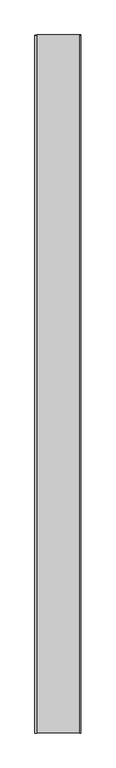
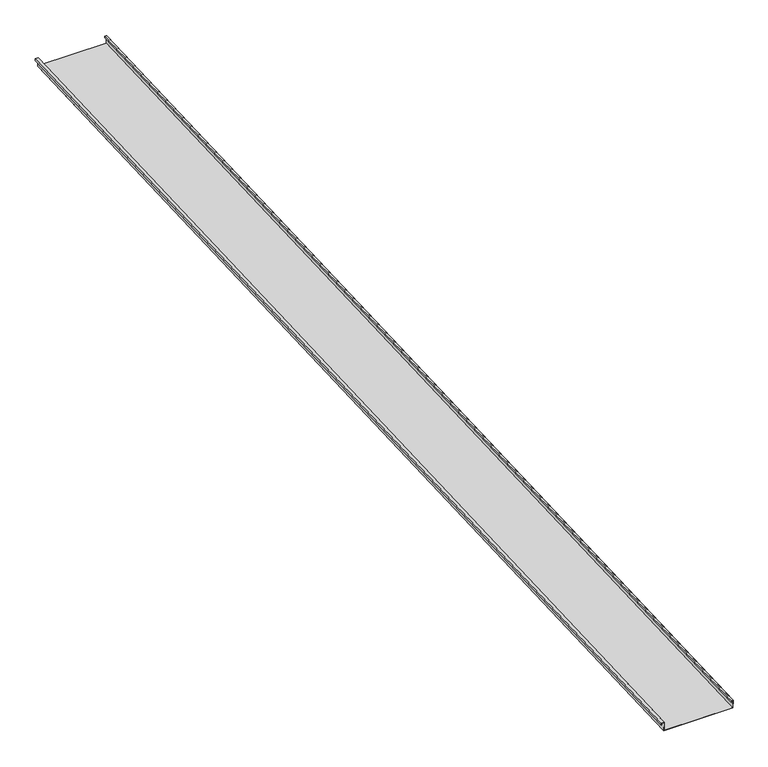
"""IFC4 building model written with IfcOpenShell, lengths in millimetres: proxy geometry, Generic Models 2:Generic Models 2:310765:Generic Models 2:310765 : Generic Models 2:Generic Models 2:310765:98 : Generic Models 2:Generic Models 2:310765:Generic Models 2:310765 : Generic Models 2:Generic Models 2:310765:300385."""

from ifc_helpers import new_model, si_unit, frame, origin, place, context, project, spatial, polyline, outline, extrude, source, transform, mapped, element, save


def generic_models_cb29957e(model_context):
    return source(origin(), model_context, "Body", "SweptSolid", [
        extrude(outline(polyline([(1.5875, 0.0), (1.5875, 50.8), (407.9875, 50.8), (407.9875, 1.5875), (396.875, 1.5875), (396.875, 11.1125), (398.4625, 11.1125), (398.4625, 3.175), (406.4, 3.175), (406.4, 49.2125), (3.175, 49.2125), (3.175, -1.5874999), (-14.2875, -1.5874999), (-14.2875, 9.525), (-12.7, 9.525), (-12.7, 0.0), (1.5875, 0.0)])), frame((613962.0429739, -581354.4345603, 3902.6697972), z_axis=(0.0, 0.9991330730923568, 0.041630544712067834), x_axis=(1.0, 0.0, 0.0)), (0.0, 0.0, 1.0), 6400.8),
    ])


if __name__ == "__main__":
    model = new_model("IFC4")
    model_context = context("Model", 3, world=origin())
    ifc_project = project(units=[si_unit("LENGTHUNIT", "METRE", prefix="MILLI")], contexts=[model_context])
    site = spatial("IfcSite", under=ifc_project)
    building = spatial("IfcBuilding", under=site)
    placement = place(None, origin())
    generic_models_shape = generic_models_cb29957e(model_context)
    element("IfcBuildingElementProxy", 1, Name="Generic Models 2:Generic Models 2:310765:Generic Models 2:310765 : Generic Models 2:Generic Models 2:310765:98 : Generic Models 2:Generic Models 2:310765:Generic Models 2:310765 : Generic Models 2:Generic Models 2:310765:300385", ObjectType="Generic Models 2:Generic Models 2:310765:Generic Models 2:310765 : Generic Models 2:Generic Models 2:310765:98 : Generic Models 2:Generic Models 2:310765:Generic Models 2:310765 : Generic Models 2:Generic Models 2:310765:300385", at=placement, inside=building, context=model_context, shape_type="MappedRepresentation", body=[
        mapped(generic_models_shape, transform((0.0, 0.0, 0.0), x_axis=(1.0, 0.0, 0.0), y_axis=(0.0, 1.0, 0.0), z_axis=(0.0, 0.0, 1.0))),
    ])
    save(model, "model.ifc")

# Revit data of these elements
# Type "Generic Models 2:Generic Models 2:310765:Generic Models 2:310765 : Generic Models 2:Generic Models 2:310765:98 : Generic Models 2:Generic Models 2:310765:Generic Models 2:310765 : Generic Models 2:Generic Models 2:310765:300385"
#   NameOverride = "Generic Models 2:Generic Models 2:310765:Generic Models 2:310765 : Generic Models 2:Generic Models 2:310765:300385"
#   ObjectTypeOverride = "Generic Models 2:310765 : Generic Models 2:Generic Models 2:310765"
#   Reference = "Generic Models 2"
#   Tag = "300385"
# Element 1 (IfcBuildingElementProxy, "Generic Models 2:Generic Models 2:310765:Generic Models 2:310765 : Generic Models 2:Generic Models 2:310765:98 : Generic Models 2:Generic Models 2:310765:Generic Models 2:310765 : Generic Models 2:Generic Models 2:310765:300385")
#   Materials on its faces: "THERMAL BROKEN ALUMINUM STOREFRONT FOR POLYCARBONATE"
# Materials
#   "THERMAL BROKEN ALUMINUM STOREFRONT FOR POLYCARBONATE": class "Unassigned", colour RGB 244 244 244, transparency 0, Keynote = "M07611300.01", Cost = 0
